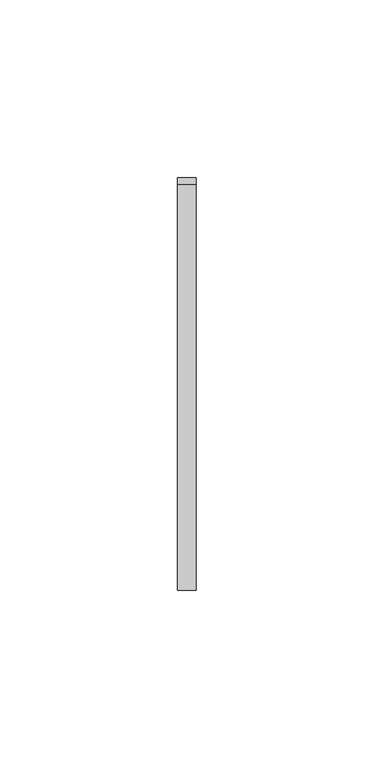
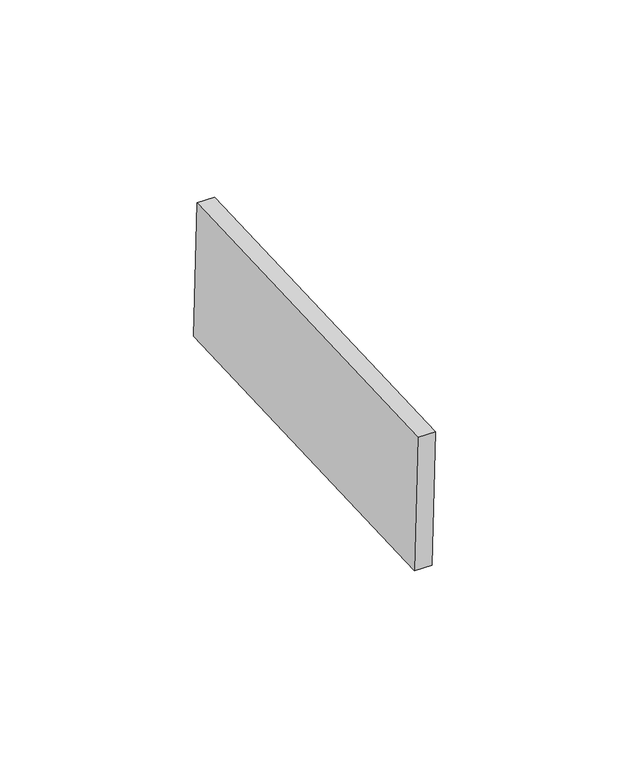
"""IFC4 building model written with IfcOpenShell, lengths in millimetres: proxy geometry, Inner panel:Inner panel:1:Inner panel:1 : Inner panel:Inner panel:300324:2:Inner panel:1:Inner panel:1 : Inner panel:Inner panel:300324:2 : Inner panel:Inner panel:1:Inner panel:1 : Inner panel:Inner panel:300324:300043:69 : Inner panel:Inner panel:1:Inner panel:1 : Inner panel:Inner panel:300324:2:Inner panel:1:Inner panel:1 : Inner panel:Inner panel:300324:2 : Inner panel:Inner panel:1:Inner panel:1 : Inner panel:Inner panel:300324:300043:308120."""

from ifc_helpers import new_model, si_unit, frame, origin, place, context, project, spatial, polyline, outline, extrude, source, transform, mapped, element, save


def generic_models_0bd7b192(model_context):
    return source(origin(), model_context, "Body", "SweptSolid", [
        extrude(outline(polyline([(0.0, -114.3), (0.0, 0.0), (5.2138089, 0.0), (5.2138089, -114.3), (0.0, -114.3)])), frame((593936.595117, -577458.3096573, 4016.6427799), z_axis=(0.0, -0.04163054471216399, 0.9991330730923527), x_axis=(-1.0, 0.0, 0.0)), (0.0, 0.0, 1.0), 43.2233908),
    ])


if __name__ == "__main__":
    model = new_model("IFC4")
    model_context = context("Model", 3, world=origin())
    ifc_project = project(units=[si_unit("LENGTHUNIT", "METRE", prefix="MILLI")], contexts=[model_context])
    site = spatial("IfcSite", under=ifc_project)
    building = spatial("IfcBuilding", under=site)
    placement = place(None, origin())
    generic_models_shape = generic_models_0bd7b192(model_context)
    element("IfcBuildingElementProxy", 1, Name="Inner panel:Inner panel:1:Inner panel:1 : Inner panel:Inner panel:300324:2:Inner panel:1:Inner panel:1 : Inner panel:Inner panel:300324:2 : Inner panel:Inner panel:1:Inner panel:1 : Inner panel:Inner panel:300324:300043:69 : Inner panel:Inner panel:1:Inner panel:1 : Inner panel:Inner panel:300324:2:Inner panel:1:Inner panel:1 : Inner panel:Inner panel:300324:2 : Inner panel:Inner panel:1:Inner panel:1 : Inner panel:Inner panel:300324:300043:308120", ObjectType="Inner panel:Inner panel:1:Inner panel:1 : Inner panel:Inner panel:300324:2:Inner panel:1:Inner panel:1 : Inner panel:Inner panel:300324:2 : Inner panel:Inner panel:1:Inner panel:1 : Inner panel:Inner panel:300324:300043:69 : Inner panel:Inner panel:1:Inner panel:1 : Inner panel:Inner panel:300324:2:Inner panel:1:Inner panel:1 : Inner panel:Inner panel:300324:2 : Inner panel:Inner panel:1:Inner panel:1 : Inner panel:Inner panel:300324:300043:308120", at=placement, inside=building, context=model_context, shape_type="MappedRepresentation", body=[
        mapped(generic_models_shape, transform((0.0, 0.0, 0.0), x_axis=(1.0, 0.0, 0.0), y_axis=(0.0, 1.0, 0.0), z_axis=(0.0, 0.0, 1.0))),
    ])
    save(model, "model.ifc")

# Revit data of these elements
# Type "Inner panel:Inner panel:1:Inner panel:1 : Inner panel:Inner panel:300324:2:Inner panel:1:Inner panel:1 : Inner panel:Inner panel:300324:2 : Inner panel:Inner panel:1:Inner panel:1 : Inner panel:Inner panel:300324:300043:69 : Inner panel:Inner panel:1:Inner panel:1 : Inner panel:Inner panel:300324:2:Inner panel:1:Inner panel:1 : Inner panel:Inner panel:300324:2 : Inner panel:Inner panel:1:Inner panel:1 : Inner panel:Inner panel:300324:300043:308120"
#   NameOverride = "Inner panel:Inner panel:1:Inner panel:1 : Inner panel:Inner panel:300324:2:Inner panel:1:Inner panel:1 : Inner panel:Inner panel:300324:2 : Inner panel:Inner panel:1:Inner panel:1 : Inner panel:Inner panel:300324:300043:308120"
#   ObjectTypeOverride = "Inner panel:1:Inner panel:1 : Inner panel:Inner panel:300324:2 : Inner panel:Inner panel:1:Inner panel:1 : Inner panel:Inner panel:300324:300043"
#   Reference = "Inner panel"
#   Tag = "308120"
# Element 1 (IfcBuildingElementProxy, "Inner panel:Inner panel:1:Inner panel:1 : Inner panel:Inner panel:300324:2:Inner panel:1:Inner panel:1 : Inner panel:Inner panel:300324:2 : Inner panel:Inner panel:1:Inner panel:1 : Inner panel:Inner panel:300324:300043:69 : Inner panel:Inner panel:1:Inner panel:1 : Inner panel:Inner panel:300324:2:Inner panel:1:Inner panel:1 : Inner panel:Inner panel:300324:2 : Inner panel:Inner panel:1:Inner panel:1 : Inner panel:Inner panel:300324:300043:308120")
#   Materials on its faces: "SLIDING CLIP"
# Materials
#   "SLIDING CLIP": class "Generic", colour RGB 120 120 120, transparency 0, Cost = 0
